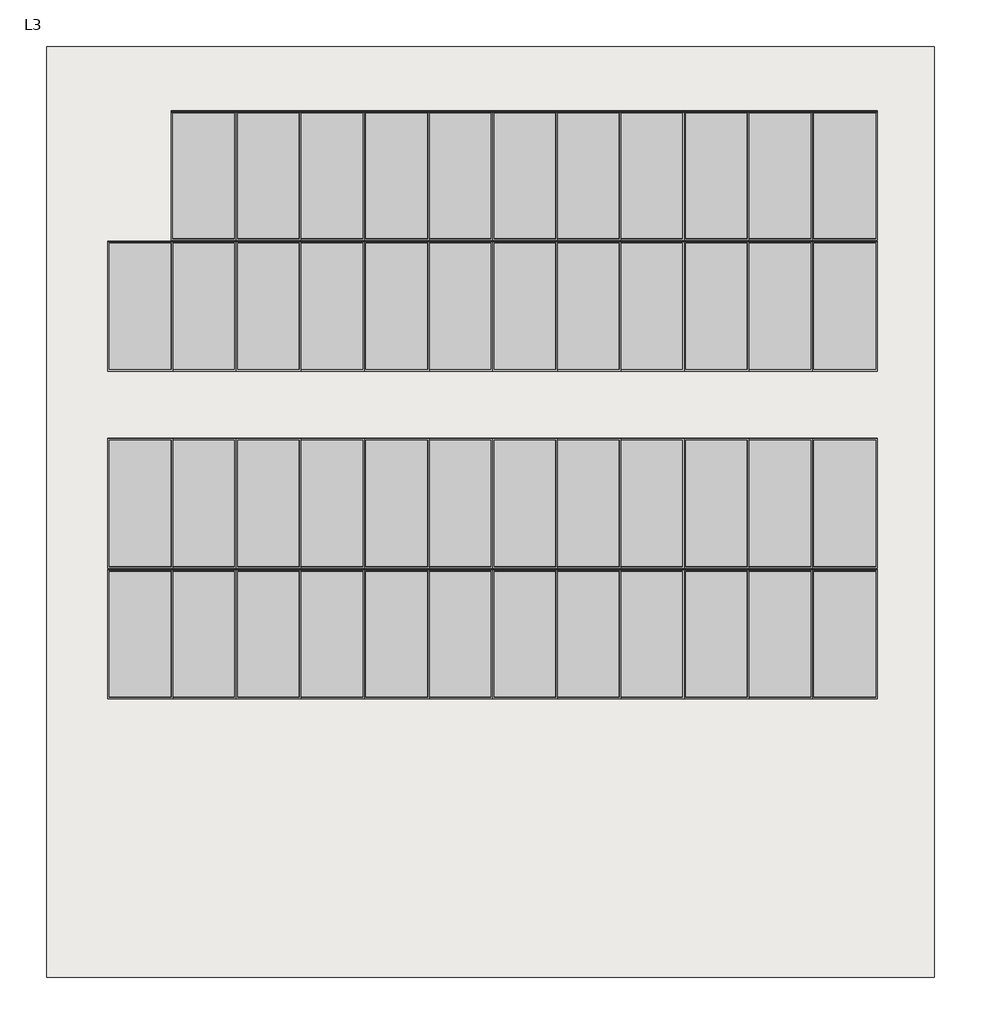
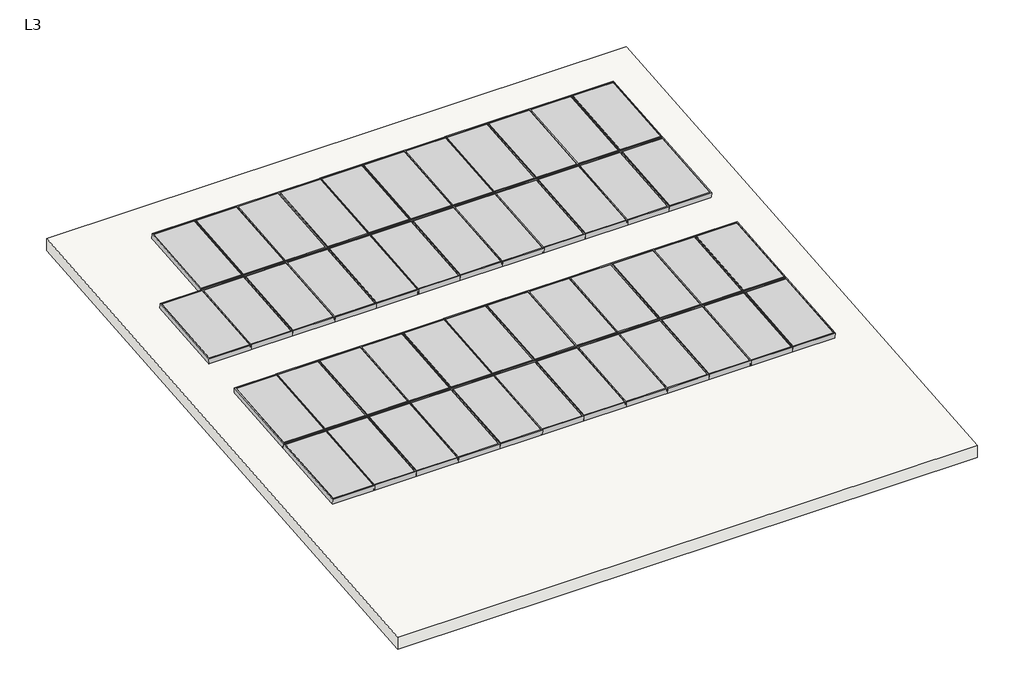
# One storey: 47 proxies, 1 roof.
"""IFC4 building model written with IfcOpenShell, lengths in millimetres."""

import ifcopenshell
import ifcopenshell.guid

model = None  # the IFC model being written
_history = None  # IfcOwnerHistory: only IFC2X3 demands one
_inside = {}  # id of a spatial element -> (the spatial element, [elements in it])
_under = {}  # id of a project, library or spatial element -> (it, [spatial elements below it])
_declared = {}  # id of a project -> (the project, [libraries it declares])
_typed = {}  # id of a type object -> (the type object, [elements of that type])
_made_of = {}  # id of a material, layer set ... -> (it, [elements and type objects made of it])


def new_model(schema):
    """Start an empty IFC model of exactly this schema.

    Asked for "IFC4X3", IfcOpenShell would pick the latest addendum, in which some entities
    have other attributes; the version numbers below select the first issue.
    IFC2X3 requires an IfcOwnerHistory on every rooted entity: one is made here for all.
    """
    global model, _history
    if schema == "IFC4X3":
        model = ifcopenshell.file(schema_version=(4, 3, 0, 0))
    else:
        model = ifcopenshell.file(schema=schema)
    _inside.clear()
    _under.clear()
    _declared.clear()
    _typed.clear()
    _made_of.clear()
    _history = None
    if model.schema == "IFC2X3":
        org = make("IfcOrganization", Name="unknown")
        user = make(
            "IfcPersonAndOrganization",
            ThePerson=make("IfcPerson", FamilyName="unknown"),
            TheOrganization=org,
        )
        app = make(
            "IfcApplication",
            ApplicationDeveloper=org,
            Version="unknown",
            ApplicationFullName="unknown",
            ApplicationIdentifier="unknown",
        )
        _history = make(
            "IfcOwnerHistory",
            OwningUser=user,
            OwningApplication=app,
            ChangeAction="ADDED",
            CreationDate=0,
        )
    return model


def make(cls, **values):
    """One entity of the class cls with the attributes given. An attribute that is None is left unset."""
    return model.create_entity(
        cls, **{name: value for name, value in values.items() if value is not None}
    )


def rooted(cls, **values):
    """An entity with a GlobalId (a new one), such as an element, a storey or a relation."""
    return make(cls, GlobalId=ifcopenshell.guid.new(), OwnerHistory=_history, **values)


def si_unit(unit_type, name, prefix=None):
    """IfcSIUnit, for example si_unit("LENGTHUNIT", "METRE", prefix="MILLI")."""
    return make("IfcSIUnit", UnitType=unit_type, Prefix=prefix, Name=name)


def assignment(units):
    """IfcUnitAssignment: the units of a project."""
    return None if units is None else make("IfcUnitAssignment", Units=units)


def point(xyz):
    """IfcCartesianPoint."""
    return None if xyz is None else make("IfcCartesianPoint", Coordinates=xyz)


def direction(xyz):
    """IfcDirection."""
    return None if xyz is None else make("IfcDirection", DirectionRatios=xyz)


def frame(location, z_axis=None, x_axis=None):
    """IfcAxis2Placement3D, a coordinate frame: its origin and axes. An axis left out is left unset."""
    return make(
        "IfcAxis2Placement3D",
        Location=point(location),
        Axis=direction(z_axis),
        RefDirection=direction(x_axis),
    )


def origin():
    """The frame at (0, 0, 0) with its axes left unset."""
    return frame((0.0, 0.0, 0.0))


def origin_with_axes():
    """The frame at (0, 0, 0) with the z axis (0, 0, 1) and the x axis (1, 0, 0) written out."""
    return frame((0.0, 0.0, 0.0), z_axis=(0.0, 0.0, 1.0), x_axis=(1.0, 0.0, 0.0))


def place(relative_to, where):
    """IfcLocalPlacement: puts the frame where relative to a parent placement (None: the world)."""
    return make(
        "IfcLocalPlacement", PlacementRelTo=relative_to, RelativePlacement=where
    )


def context(
    kind, dimensions, precision=None, world=None, true_north=None, identifier=None
):
    """IfcGeometricRepresentationContext, for example the 3D "Model" context."""
    return make(
        "IfcGeometricRepresentationContext",
        ContextIdentifier=identifier,
        ContextType=kind,
        CoordinateSpaceDimension=dimensions,
        Precision=precision,
        WorldCoordinateSystem=world,
        TrueNorth=true_north,
    )


def project(units=None, contexts=None):
    """IfcProject with its units and contexts."""
    return rooted(
        "IfcProject",
        Name="project",
        RepresentationContexts=contexts,
        UnitsInContext=assignment(units),
    )


def spatial(cls, under=None, at=None, **own):
    """A site, building, storey or space (cls), placed at a placement, below another one or the project."""
    s = rooted(cls, ObjectPlacement=at, **own)
    if under is not None:
        _under.setdefault(under.id(), (under, []))[1].append(s)
    return s


def polyline(points):
    """IfcPolyline through the points."""
    return make("IfcPolyline", Points=[point(p) for p in points])


def outline(outer, holes=None, kind="AREA"):
    """IfcArbitraryClosedProfileDef: a profile drawn as a closed curve; with holes, ...WithVoids."""
    if holes is None:
        return make("IfcArbitraryClosedProfileDef", ProfileType=kind, OuterCurve=outer)
    return make(
        "IfcArbitraryProfileDefWithVoids",
        ProfileType=kind,
        OuterCurve=outer,
        InnerCurves=holes,
    )


def extrude(swept, where, along, depth):
    """IfcExtrudedAreaSolid: the profile swept, set in the frame where, extruded along a direction by depth."""
    return make(
        "IfcExtrudedAreaSolid",
        SweptArea=swept,
        Position=where,
        ExtrudedDirection=direction(along),
        Depth=depth,
    )


def shape(context_of_items, identifier, shape_type, items):
    """IfcShapeRepresentation: the items that make up one representation, for example the "Body"."""
    return make(
        "IfcShapeRepresentation",
        ContextOfItems=context_of_items,
        RepresentationIdentifier=identifier,
        RepresentationType=shape_type,
        Items=items,
    )


def source(mapping_origin, context_of_items, identifier, shape_type, items):
    """IfcRepresentationMap: a shape defined once, which mapped items show again and again."""
    return make(
        "IfcRepresentationMap",
        MappingOrigin=mapping_origin,
        MappedRepresentation=shape(context_of_items, identifier, shape_type, items),
    )


def transform(
    local_origin,
    x_axis=None,
    y_axis=None,
    z_axis=None,
    scale=None,
    scale2=None,
    scale3=None,
    uniform=True,
):
    """IfcCartesianTransformationOperator3D, or its non-uniform kind. x_axis, y_axis, z_axis: its Axis1, 2, 3."""
    if uniform:
        return make(
            "IfcCartesianTransformationOperator3D",
            Axis1=direction(x_axis),
            Axis2=direction(y_axis),
            LocalOrigin=point(local_origin),
            Scale=scale,
            Axis3=direction(z_axis),
        )
    return make(
        "IfcCartesianTransformationOperator3DnonUniform",
        Axis1=direction(x_axis),
        Axis2=direction(y_axis),
        LocalOrigin=point(local_origin),
        Scale=scale,
        Axis3=direction(z_axis),
        Scale2=scale2,
        Scale3=scale3,
    )


def mapped(mapping_source, mapping_target):
    """IfcMappedItem: shows the shape of a source again, moved by a transform."""
    return make(
        "IfcMappedItem", MappingSource=mapping_source, MappingTarget=mapping_target
    )


def made_of(thing, what):
    """Note that an element or type object is made of a material, layer set ...; save() writes the relation."""
    if what is not None:
        _made_of.setdefault(what.id(), (what, []))[1].append(thing)
    return thing


def element(
    cls,
    number,
    at=None,
    inside=None,
    cuts=None,
    type_object=None,
    material=None,
    context=None,
    identifier="Body",
    shape_type=None,
    held_by="IfcProductDefinitionShape",
    body=None,
    shapes=None,
    **own,
):
    """One element of the class cls, such as IfcWall. Its Tag is "e" and its number.

    at: its placement. inside: the storey or other place that contains it. cuts: it is an
    opening in that element (IfcRelVoidsElement). A single representation is given by context,
    identifier, shape_type and body (its items); several are given by shapes. held_by: the class
    of the entity that holds the representations. save() writes the other relations.
    """
    e = rooted(cls, Tag="e%d" % number, ObjectPlacement=at, **own)
    if body is not None:
        shapes = [shape(context, identifier, shape_type, body)]
    if shapes is not None:
        e.Representation = make(held_by, Representations=shapes)
    if inside is not None:
        _inside.setdefault(inside.id(), (inside, []))[1].append(e)
    if cuts is not None:
        rooted(
            "IfcRelVoidsElement", RelatingBuildingElement=cuts, RelatedOpeningElement=e
        )
    if type_object is not None:
        _typed.setdefault(type_object.id(), (type_object, []))[1].append(e)
    return made_of(e, material)


def aggregate(whole, parts):
    """IfcRelAggregates: a whole, such as a stair, and the parts it consists of."""
    return rooted("IfcRelAggregates", RelatingObject=whole, RelatedObjects=parts)


def save(model, path):
    """Write the relations noted so far, then the file.

    IfcRelAggregates (storeys below a building ...), IfcRelContainedInSpatialStructure (elements
    in a storey), IfcRelDefinesByType, IfcRelAssociatesMaterial and IfcRelDeclares: one each for
    every whole, place, type object, material and project.
    """
    for whole, parts in _under.values():
        aggregate(whole, parts)
    for where, things in _inside.values():
        rooted(
            "IfcRelContainedInSpatialStructure",
            RelatedElements=things,
            RelatingStructure=where,
        )
    for kind, things in _typed.values():
        rooted("IfcRelDefinesByType", RelatedObjects=things, RelatingType=kind)
    for what, things in _made_of.values():
        rooted("IfcRelAssociatesMaterial", RelatedObjects=things, RelatingMaterial=what)
    for by, libraries in _declared.values():
        rooted("IfcRelDeclares", RelatingContext=by, RelatedDefinitions=libraries)
    model.write(path)


def m_solar_panel_750_x_1500mm_21fb4d5c(model_context):
    return source(origin(), model_context, "Body", "SweptSolid", [
        extrude(outline(polyline([(32.32, 1500.0), (782.32, 1500.0), (782.32, 0.0), (32.32, 0.0), (32.32, 1500.0)]), holes=[polyline([(763.27, 1480.95), (51.37, 1480.95), (51.37, 19.05), (763.27, 19.05), (763.27, 1480.95)])]), origin_with_axes(), (0.0, 0.0, 1.0), 100.0),
        extrude(outline(polyline([(763.27, 1480.95), (763.27, 19.05), (51.37, 19.05), (51.37, 1480.95), (763.27, 1480.95)])), origin_with_axes(), (0.0, 0.0, 1.0), 93.65),
    ])


model = new_model("IFC4")

# Units and contexts
model_context = context("Model", 3, world=origin())
ifc_project = project(units=[si_unit("LENGTHUNIT", "METRE", prefix="MILLI")], contexts=[model_context])

# Site, building, storey
site = spatial("IfcSite", under=ifc_project)
building = spatial("IfcBuilding", under=site)
storey = spatial("IfcBuildingStorey", under=building, Name="L3", Elevation=6000.0)

# Proxies
placement = place(None, origin())
m_solar_panel_750_x_1500mm_shape = m_solar_panel_750_x_1500mm_21fb4d5c(model_context)
element("IfcBuildingElementProxy", 1, Name="M_Solar Panel : 750 x 1500mm", ObjectType="M_Solar Panel : 750 x 1500mm", at=placement, inside=storey, context=model_context, shape_type="MappedRepresentation", body=[
    mapped(m_solar_panel_750_x_1500mm_shape, transform((-3719.703333, 2644.8337429, 6971.2483311), x_axis=(1.0, 0.0, 0.0), y_axis=(0.0, 0.9961946980917455, 0.08715574274765815), z_axis=(0.0, -0.08715574274765815, 0.9961946980917455))),
])
element("IfcBuildingElementProxy", 2, Name="M_Solar Panel : 750 x 1500mm", ObjectType="M_Solar Panel : 750 x 1500mm", at=placement, inside=storey, context=model_context, shape_type="MappedRepresentation", body=[
    mapped(m_solar_panel_750_x_1500mm_shape, transform((-2969.703333, 2644.8337429, 6971.2483311), x_axis=(1.0, 0.0, 0.0), y_axis=(0.0, 0.9961946980917455, 0.08715574274765815), z_axis=(0.0, -0.08715574274765815, 0.9961946980917455))),
])
element("IfcBuildingElementProxy", 3, Name="M_Solar Panel : 750 x 1500mm", ObjectType="M_Solar Panel : 750 x 1500mm", at=placement, inside=storey, context=model_context, shape_type="MappedRepresentation", body=[
    mapped(m_solar_panel_750_x_1500mm_shape, transform((-2238.753333, 2644.8337429, 6971.2483311), x_axis=(1.0, 0.0, 0.0), y_axis=(0.0, 0.9961946980917455, 0.08715574274765815), z_axis=(0.0, -0.08715574274765815, 0.9961946980917455))),
])
element("IfcBuildingElementProxy", 4, Name="M_Solar Panel : 750 x 1500mm", ObjectType="M_Solar Panel : 750 x 1500mm", at=placement, inside=storey, context=model_context, shape_type="MappedRepresentation", body=[
    mapped(m_solar_panel_750_x_1500mm_shape, transform((-1488.753333, 2644.8337429, 6971.2483311), x_axis=(1.0, 0.0, 0.0), y_axis=(0.0, 0.9961946980917455, 0.08715574274765815), z_axis=(0.0, -0.08715574274765815, 0.9961946980917455))),
])
element("IfcBuildingElementProxy", 5, Name="M_Solar Panel : 750 x 1500mm", ObjectType="M_Solar Panel : 750 x 1500mm", at=placement, inside=storey, context=model_context, shape_type="MappedRepresentation", body=[
    mapped(m_solar_panel_750_x_1500mm_shape, transform((-757.803333, 2644.8337429, 6971.2483311), x_axis=(1.0, 0.0, 0.0), y_axis=(0.0, 0.9961946980917455, 0.08715574274765815), z_axis=(0.0, -0.08715574274765815, 0.9961946980917455))),
])
element("IfcBuildingElementProxy", 6, Name="M_Solar Panel : 750 x 1500mm", ObjectType="M_Solar Panel : 750 x 1500mm", at=placement, inside=storey, context=model_context, shape_type="MappedRepresentation", body=[
    mapped(m_solar_panel_750_x_1500mm_shape, transform((-7.803333, 2644.8337429, 6971.2483311), x_axis=(1.0, 0.0, 0.0), y_axis=(0.0, 0.9961946980917455, 0.08715574274765815), z_axis=(0.0, -0.08715574274765815, 0.9961946980917455))),
])
element("IfcBuildingElementProxy", 7, Name="M_Solar Panel : 750 x 1500mm", ObjectType="M_Solar Panel : 750 x 1500mm", at=placement, inside=storey, context=model_context, shape_type="MappedRepresentation", body=[
    mapped(m_solar_panel_750_x_1500mm_shape, transform((723.146667, 2644.8337429, 6971.2483311), x_axis=(1.0, 0.0, 0.0), y_axis=(0.0, 0.9961946980917455, 0.08715574274765815), z_axis=(0.0, -0.08715574274765815, 0.9961946980917455))),
])
element("IfcBuildingElementProxy", 8, Name="M_Solar Panel : 750 x 1500mm", ObjectType="M_Solar Panel : 750 x 1500mm", at=placement, inside=storey, context=model_context, shape_type="MappedRepresentation", body=[
    mapped(m_solar_panel_750_x_1500mm_shape, transform((1454.096667, 2644.8337429, 6971.2483311), x_axis=(1.0, 0.0, 0.0), y_axis=(0.0, 0.9961946980917455, 0.08715574274765815), z_axis=(0.0, -0.08715574274765815, 0.9961946980917455))),
])
element("IfcBuildingElementProxy", 9, Name="M_Solar Panel : 750 x 1500mm", ObjectType="M_Solar Panel : 750 x 1500mm", at=placement, inside=storey, context=model_context, shape_type="MappedRepresentation", body=[
    mapped(m_solar_panel_750_x_1500mm_shape, transform((2204.096667, 2644.8337429, 6971.2483311), x_axis=(1.0, 0.0, 0.0), y_axis=(0.0, 0.9961946980917455, 0.08715574274765815), z_axis=(0.0, -0.08715574274765815, 0.9961946980917455))),
])
element("IfcBuildingElementProxy", 10, Name="M_Solar Panel : 750 x 1500mm", ObjectType="M_Solar Panel : 750 x 1500mm", at=placement, inside=storey, context=model_context, shape_type="MappedRepresentation", body=[
    mapped(m_solar_panel_750_x_1500mm_shape, transform((2935.046667, 2644.8337429, 6971.2483311), x_axis=(1.0, 0.0, 0.0), y_axis=(0.0, 0.9961946980917455, 0.08715574274765815), z_axis=(0.0, -0.08715574274765815, 0.9961946980917455))),
])
element("IfcBuildingElementProxy", 11, Name="M_Solar Panel : 750 x 1500mm", ObjectType="M_Solar Panel : 750 x 1500mm", at=placement, inside=storey, context=model_context, shape_type="MappedRepresentation", body=[
    mapped(m_solar_panel_750_x_1500mm_shape, transform((3685.046667, 2644.8337429, 6971.2483311), x_axis=(1.0, 0.0, 0.0), y_axis=(0.0, 0.9961946980917455, 0.08715574274765815), z_axis=(0.0, -0.08715574274765815, 0.9961946980917455))),
])
element("IfcBuildingElementProxy", 12, Name="M_Solar Panel : 750 x 1500mm", ObjectType="M_Solar Panel : 750 x 1500mm", at=placement, inside=storey, context=model_context, shape_type="MappedRepresentation", body=[
    mapped(m_solar_panel_750_x_1500mm_shape, transform((-4450.653333, 1135.5987753, 6839.2073808), x_axis=(1.0, 0.0, 0.0), y_axis=(0.0, 0.9961946980917455, 0.08715574274765815), z_axis=(0.0, -0.08715574274765815, 0.9961946980917455))),
])
element("IfcBuildingElementProxy", 13, Name="M_Solar Panel : 750 x 1500mm", ObjectType="M_Solar Panel : 750 x 1500mm", at=placement, inside=storey, context=model_context, shape_type="MappedRepresentation", body=[
    mapped(m_solar_panel_750_x_1500mm_shape, transform((-3719.703333, 1135.5987753, 6839.2073808), x_axis=(1.0, 0.0, 0.0), y_axis=(0.0, 0.9961946980917455, 0.08715574274765815), z_axis=(0.0, -0.08715574274765815, 0.9961946980917455))),
])
element("IfcBuildingElementProxy", 14, Name="M_Solar Panel : 750 x 1500mm", ObjectType="M_Solar Panel : 750 x 1500mm", at=placement, inside=storey, context=model_context, shape_type="MappedRepresentation", body=[
    mapped(m_solar_panel_750_x_1500mm_shape, transform((-2969.703333, 1135.5987753, 6839.2073808), x_axis=(1.0, 0.0, 0.0), y_axis=(0.0, 0.9961946980917455, 0.08715574274765815), z_axis=(0.0, -0.08715574274765815, 0.9961946980917455))),
])
element("IfcBuildingElementProxy", 15, Name="M_Solar Panel : 750 x 1500mm", ObjectType="M_Solar Panel : 750 x 1500mm", at=placement, inside=storey, context=model_context, shape_type="MappedRepresentation", body=[
    mapped(m_solar_panel_750_x_1500mm_shape, transform((-2238.753333, 1135.5987753, 6839.2073808), x_axis=(1.0, 0.0, 0.0), y_axis=(0.0, 0.9961946980917455, 0.08715574274765815), z_axis=(0.0, -0.08715574274765815, 0.9961946980917455))),
])
element("IfcBuildingElementProxy", 16, Name="M_Solar Panel : 750 x 1500mm", ObjectType="M_Solar Panel : 750 x 1500mm", at=placement, inside=storey, context=model_context, shape_type="MappedRepresentation", body=[
    mapped(m_solar_panel_750_x_1500mm_shape, transform((-1488.753333, 1135.5987753, 6839.2073808), x_axis=(1.0, 0.0, 0.0), y_axis=(0.0, 0.9961946980917455, 0.08715574274765815), z_axis=(0.0, -0.08715574274765815, 0.9961946980917455))),
])
element("IfcBuildingElementProxy", 17, Name="M_Solar Panel : 750 x 1500mm", ObjectType="M_Solar Panel : 750 x 1500mm", at=placement, inside=storey, context=model_context, shape_type="MappedRepresentation", body=[
    mapped(m_solar_panel_750_x_1500mm_shape, transform((-757.803333, 1135.5987753, 6839.2073808), x_axis=(1.0, 0.0, 0.0), y_axis=(0.0, 0.9961946980917455, 0.08715574274765815), z_axis=(0.0, -0.08715574274765815, 0.9961946980917455))),
])
element("IfcBuildingElementProxy", 18, Name="M_Solar Panel : 750 x 1500mm", ObjectType="M_Solar Panel : 750 x 1500mm", at=placement, inside=storey, context=model_context, shape_type="MappedRepresentation", body=[
    mapped(m_solar_panel_750_x_1500mm_shape, transform((-7.803333, 1135.5987753, 6839.2073808), x_axis=(1.0, 0.0, 0.0), y_axis=(0.0, 0.9961946980917455, 0.08715574274765815), z_axis=(0.0, -0.08715574274765815, 0.9961946980917455))),
])
element("IfcBuildingElementProxy", 19, Name="M_Solar Panel : 750 x 1500mm", ObjectType="M_Solar Panel : 750 x 1500mm", at=placement, inside=storey, context=model_context, shape_type="MappedRepresentation", body=[
    mapped(m_solar_panel_750_x_1500mm_shape, transform((723.146667, 1135.5987753, 6839.2073808), x_axis=(1.0, 0.0, 0.0), y_axis=(0.0, 0.9961946980917455, 0.08715574274765815), z_axis=(0.0, -0.08715574274765815, 0.9961946980917455))),
])
element("IfcBuildingElementProxy", 20, Name="M_Solar Panel : 750 x 1500mm", ObjectType="M_Solar Panel : 750 x 1500mm", at=placement, inside=storey, context=model_context, shape_type="MappedRepresentation", body=[
    mapped(m_solar_panel_750_x_1500mm_shape, transform((1454.096667, 1135.5987753, 6839.2073808), x_axis=(1.0, 0.0, 0.0), y_axis=(0.0, 0.9961946980917455, 0.08715574274765815), z_axis=(0.0, -0.08715574274765815, 0.9961946980917455))),
])
element("IfcBuildingElementProxy", 21, Name="M_Solar Panel : 750 x 1500mm", ObjectType="M_Solar Panel : 750 x 1500mm", at=placement, inside=storey, context=model_context, shape_type="MappedRepresentation", body=[
    mapped(m_solar_panel_750_x_1500mm_shape, transform((2204.096667, 1135.5987753, 6839.2073808), x_axis=(1.0, 0.0, 0.0), y_axis=(0.0, 0.9961946980917455, 0.08715574274765815), z_axis=(0.0, -0.08715574274765815, 0.9961946980917455))),
])
element("IfcBuildingElementProxy", 22, Name="M_Solar Panel : 750 x 1500mm", ObjectType="M_Solar Panel : 750 x 1500mm", at=placement, inside=storey, context=model_context, shape_type="MappedRepresentation", body=[
    mapped(m_solar_panel_750_x_1500mm_shape, transform((2935.046667, 1135.5987753, 6839.2073808), x_axis=(1.0, 0.0, 0.0), y_axis=(0.0, 0.9961946980917455, 0.08715574274765815), z_axis=(0.0, -0.08715574274765815, 0.9961946980917455))),
])
element("IfcBuildingElementProxy", 23, Name="M_Solar Panel : 750 x 1500mm", ObjectType="M_Solar Panel : 750 x 1500mm", at=placement, inside=storey, context=model_context, shape_type="MappedRepresentation", body=[
    mapped(m_solar_panel_750_x_1500mm_shape, transform((3685.046667, 1135.5987753, 6839.2073808), x_axis=(1.0, 0.0, 0.0), y_axis=(0.0, 0.9961946980917455, 0.08715574274765815), z_axis=(0.0, -0.08715574274765815, 0.9961946980917455))),
])
element("IfcBuildingElementProxy", 24, Name="M_Solar Panel : 750 x 1500mm", ObjectType="M_Solar Panel : 750 x 1500mm", at=placement, inside=storey, context=model_context, shape_type="MappedRepresentation", body=[
    mapped(m_solar_panel_750_x_1500mm_shape, transform((-4450.653333, -1140.7061098, 6640.0565086), x_axis=(1.0, 0.0, 0.0), y_axis=(0.0, 0.9961946980917455, 0.08715574274765815), z_axis=(0.0, -0.08715574274765815, 0.9961946980917455))),
])
element("IfcBuildingElementProxy", 25, Name="M_Solar Panel : 750 x 1500mm", ObjectType="M_Solar Panel : 750 x 1500mm", at=placement, inside=storey, context=model_context, shape_type="MappedRepresentation", body=[
    mapped(m_solar_panel_750_x_1500mm_shape, transform((-3719.703333, -1140.7061098, 6640.0565086), x_axis=(1.0, 0.0, 0.0), y_axis=(0.0, 0.9961946980917455, 0.08715574274765815), z_axis=(0.0, -0.08715574274765815, 0.9961946980917455))),
])
element("IfcBuildingElementProxy", 26, Name="M_Solar Panel : 750 x 1500mm", ObjectType="M_Solar Panel : 750 x 1500mm", at=placement, inside=storey, context=model_context, shape_type="MappedRepresentation", body=[
    mapped(m_solar_panel_750_x_1500mm_shape, transform((-2969.703333, -1140.7061098, 6640.0565086), x_axis=(1.0, 0.0, 0.0), y_axis=(0.0, 0.9961946980917455, 0.08715574274765815), z_axis=(0.0, -0.08715574274765815, 0.9961946980917455))),
])
element("IfcBuildingElementProxy", 27, Name="M_Solar Panel : 750 x 1500mm", ObjectType="M_Solar Panel : 750 x 1500mm", at=placement, inside=storey, context=model_context, shape_type="MappedRepresentation", body=[
    mapped(m_solar_panel_750_x_1500mm_shape, transform((-2238.753333, -1140.7061098, 6640.0565086), x_axis=(1.0, 0.0, 0.0), y_axis=(0.0, 0.9961946980917455, 0.08715574274765815), z_axis=(0.0, -0.08715574274765815, 0.9961946980917455))),
])
element("IfcBuildingElementProxy", 28, Name="M_Solar Panel : 750 x 1500mm", ObjectType="M_Solar Panel : 750 x 1500mm", at=placement, inside=storey, context=model_context, shape_type="MappedRepresentation", body=[
    mapped(m_solar_panel_750_x_1500mm_shape, transform((-1488.753333, -1140.7061098, 6640.0565086), x_axis=(1.0, 0.0, 0.0), y_axis=(0.0, 0.9961946980917455, 0.08715574274765815), z_axis=(0.0, -0.08715574274765815, 0.9961946980917455))),
])
element("IfcBuildingElementProxy", 29, Name="M_Solar Panel : 750 x 1500mm", ObjectType="M_Solar Panel : 750 x 1500mm", at=placement, inside=storey, context=model_context, shape_type="MappedRepresentation", body=[
    mapped(m_solar_panel_750_x_1500mm_shape, transform((-757.803333, -1140.7061098, 6640.0565086), x_axis=(1.0, 0.0, 0.0), y_axis=(0.0, 0.9961946980917455, 0.08715574274765815), z_axis=(0.0, -0.08715574274765815, 0.9961946980917455))),
])
element("IfcBuildingElementProxy", 30, Name="M_Solar Panel : 750 x 1500mm", ObjectType="M_Solar Panel : 750 x 1500mm", at=placement, inside=storey, context=model_context, shape_type="MappedRepresentation", body=[
    mapped(m_solar_panel_750_x_1500mm_shape, transform((-7.803333, -1140.7061098, 6640.0565086), x_axis=(1.0, 0.0, 0.0), y_axis=(0.0, 0.9961946980917455, 0.08715574274765815), z_axis=(0.0, -0.08715574274765815, 0.9961946980917455))),
])
element("IfcBuildingElementProxy", 31, Name="M_Solar Panel : 750 x 1500mm", ObjectType="M_Solar Panel : 750 x 1500mm", at=placement, inside=storey, context=model_context, shape_type="MappedRepresentation", body=[
    mapped(m_solar_panel_750_x_1500mm_shape, transform((723.146667, -1140.7061098, 6640.0565086), x_axis=(1.0, 0.0, 0.0), y_axis=(0.0, 0.9961946980917455, 0.08715574274765815), z_axis=(0.0, -0.08715574274765815, 0.9961946980917455))),
])
element("IfcBuildingElementProxy", 32, Name="M_Solar Panel : 750 x 1500mm", ObjectType="M_Solar Panel : 750 x 1500mm", at=placement, inside=storey, context=model_context, shape_type="MappedRepresentation", body=[
    mapped(m_solar_panel_750_x_1500mm_shape, transform((1454.096667, -1140.7061098, 6640.0565086), x_axis=(1.0, 0.0, 0.0), y_axis=(0.0, 0.9961946980917455, 0.08715574274765815), z_axis=(0.0, -0.08715574274765815, 0.9961946980917455))),
])
element("IfcBuildingElementProxy", 33, Name="M_Solar Panel : 750 x 1500mm", ObjectType="M_Solar Panel : 750 x 1500mm", at=placement, inside=storey, context=model_context, shape_type="MappedRepresentation", body=[
    mapped(m_solar_panel_750_x_1500mm_shape, transform((2204.096667, -1140.7061098, 6640.0565086), x_axis=(1.0, 0.0, 0.0), y_axis=(0.0, 0.9961946980917455, 0.08715574274765815), z_axis=(0.0, -0.08715574274765815, 0.9961946980917455))),
])
element("IfcBuildingElementProxy", 34, Name="M_Solar Panel : 750 x 1500mm", ObjectType="M_Solar Panel : 750 x 1500mm", at=placement, inside=storey, context=model_context, shape_type="MappedRepresentation", body=[
    mapped(m_solar_panel_750_x_1500mm_shape, transform((2935.046667, -1140.7061098, 6640.0565086), x_axis=(1.0, 0.0, 0.0), y_axis=(0.0, 0.9961946980917455, 0.08715574274765815), z_axis=(0.0, -0.08715574274765815, 0.9961946980917455))),
])
element("IfcBuildingElementProxy", 35, Name="M_Solar Panel : 750 x 1500mm", ObjectType="M_Solar Panel : 750 x 1500mm", at=placement, inside=storey, context=model_context, shape_type="MappedRepresentation", body=[
    mapped(m_solar_panel_750_x_1500mm_shape, transform((3685.046667, -1140.7061098, 6640.0565086), x_axis=(1.0, 0.0, 0.0), y_axis=(0.0, 0.9961946980917455, 0.08715574274765815), z_axis=(0.0, -0.08715574274765815, 0.9961946980917455))),
])
element("IfcBuildingElementProxy", 36, Name="M_Solar Panel : 750 x 1500mm", ObjectType="M_Solar Panel : 750 x 1500mm", at=placement, inside=storey, context=model_context, shape_type="MappedRepresentation", body=[
    mapped(m_solar_panel_750_x_1500mm_shape, transform((-4450.653333, -2649.9410774, 6508.0155584), x_axis=(1.0, 0.0, 0.0), y_axis=(0.0, 0.9961946980917455, 0.08715574274765815), z_axis=(0.0, -0.08715574274765815, 0.9961946980917455))),
])
element("IfcBuildingElementProxy", 37, Name="M_Solar Panel : 750 x 1500mm", ObjectType="M_Solar Panel : 750 x 1500mm", at=placement, inside=storey, context=model_context, shape_type="MappedRepresentation", body=[
    mapped(m_solar_panel_750_x_1500mm_shape, transform((-3719.703333, -2649.9410774, 6508.0155584), x_axis=(1.0, 0.0, 0.0), y_axis=(0.0, 0.9961946980917455, 0.08715574274765815), z_axis=(0.0, -0.08715574274765815, 0.9961946980917455))),
])
element("IfcBuildingElementProxy", 38, Name="M_Solar Panel : 750 x 1500mm", ObjectType="M_Solar Panel : 750 x 1500mm", at=placement, inside=storey, context=model_context, shape_type="MappedRepresentation", body=[
    mapped(m_solar_panel_750_x_1500mm_shape, transform((-2969.703333, -2649.9410774, 6508.0155584), x_axis=(1.0, 0.0, 0.0), y_axis=(0.0, 0.9961946980917455, 0.08715574274765815), z_axis=(0.0, -0.08715574274765815, 0.9961946980917455))),
])
element("IfcBuildingElementProxy", 39, Name="M_Solar Panel : 750 x 1500mm", ObjectType="M_Solar Panel : 750 x 1500mm", at=placement, inside=storey, context=model_context, shape_type="MappedRepresentation", body=[
    mapped(m_solar_panel_750_x_1500mm_shape, transform((-2238.753333, -2649.9410774, 6508.0155584), x_axis=(1.0, 0.0, 0.0), y_axis=(0.0, 0.9961946980917455, 0.08715574274765815), z_axis=(0.0, -0.08715574274765815, 0.9961946980917455))),
])
element("IfcBuildingElementProxy", 40, Name="M_Solar Panel : 750 x 1500mm", ObjectType="M_Solar Panel : 750 x 1500mm", at=placement, inside=storey, context=model_context, shape_type="MappedRepresentation", body=[
    mapped(m_solar_panel_750_x_1500mm_shape, transform((-1488.753333, -2649.9410774, 6508.0155584), x_axis=(1.0, 0.0, 0.0), y_axis=(0.0, 0.9961946980917455, 0.08715574274765815), z_axis=(0.0, -0.08715574274765815, 0.9961946980917455))),
])
element("IfcBuildingElementProxy", 41, Name="M_Solar Panel : 750 x 1500mm", ObjectType="M_Solar Panel : 750 x 1500mm", at=placement, inside=storey, context=model_context, shape_type="MappedRepresentation", body=[
    mapped(m_solar_panel_750_x_1500mm_shape, transform((-757.803333, -2649.9410774, 6508.0155584), x_axis=(1.0, 0.0, 0.0), y_axis=(0.0, 0.9961946980917455, 0.08715574274765815), z_axis=(0.0, -0.08715574274765815, 0.9961946980917455))),
])
element("IfcBuildingElementProxy", 42, Name="M_Solar Panel : 750 x 1500mm", ObjectType="M_Solar Panel : 750 x 1500mm", at=placement, inside=storey, context=model_context, shape_type="MappedRepresentation", body=[
    mapped(m_solar_panel_750_x_1500mm_shape, transform((-7.803333, -2649.9410774, 6508.0155584), x_axis=(1.0, 0.0, 0.0), y_axis=(0.0, 0.9961946980917455, 0.08715574274765815), z_axis=(0.0, -0.08715574274765815, 0.9961946980917455))),
])
element("IfcBuildingElementProxy", 43, Name="M_Solar Panel : 750 x 1500mm", ObjectType="M_Solar Panel : 750 x 1500mm", at=placement, inside=storey, context=model_context, shape_type="MappedRepresentation", body=[
    mapped(m_solar_panel_750_x_1500mm_shape, transform((723.146667, -2649.9410774, 6508.0155584), x_axis=(1.0, 0.0, 0.0), y_axis=(0.0, 0.9961946980917455, 0.08715574274765815), z_axis=(0.0, -0.08715574274765815, 0.9961946980917455))),
])
element("IfcBuildingElementProxy", 44, Name="M_Solar Panel : 750 x 1500mm", ObjectType="M_Solar Panel : 750 x 1500mm", at=placement, inside=storey, context=model_context, shape_type="MappedRepresentation", body=[
    mapped(m_solar_panel_750_x_1500mm_shape, transform((1454.096667, -2649.9410774, 6508.0155584), x_axis=(1.0, 0.0, 0.0), y_axis=(0.0, 0.9961946980917455, 0.08715574274765815), z_axis=(0.0, -0.08715574274765815, 0.9961946980917455))),
])
element("IfcBuildingElementProxy", 45, Name="M_Solar Panel : 750 x 1500mm", ObjectType="M_Solar Panel : 750 x 1500mm", at=placement, inside=storey, context=model_context, shape_type="MappedRepresentation", body=[
    mapped(m_solar_panel_750_x_1500mm_shape, transform((2204.096667, -2649.9410774, 6508.0155584), x_axis=(1.0, 0.0, 0.0), y_axis=(0.0, 0.9961946980917455, 0.08715574274765815), z_axis=(0.0, -0.08715574274765815, 0.9961946980917455))),
])
element("IfcBuildingElementProxy", 46, Name="M_Solar Panel : 750 x 1500mm", ObjectType="M_Solar Panel : 750 x 1500mm", at=placement, inside=storey, context=model_context, shape_type="MappedRepresentation", body=[
    mapped(m_solar_panel_750_x_1500mm_shape, transform((2935.046667, -2649.9410774, 6508.0155584), x_axis=(1.0, 0.0, 0.0), y_axis=(0.0, 0.9961946980917455, 0.08715574274765815), z_axis=(0.0, -0.08715574274765815, 0.9961946980917455))),
])
element("IfcBuildingElementProxy", 47, Name="M_Solar Panel : 750 x 1500mm", ObjectType="M_Solar Panel : 750 x 1500mm", at=placement, inside=storey, context=model_context, shape_type="MappedRepresentation", body=[
    mapped(m_solar_panel_750_x_1500mm_shape, transform((3685.046667, -2649.9410774, 6508.0155584), x_axis=(1.0, 0.0, 0.0), y_axis=(0.0, 0.9961946980917455, 0.08715574274765815), z_axis=(0.0, -0.08715574274765815, 0.9961946980917455))),
])

# Roof
element("IfcRoof", 48, ObjectType="Genérico - 225 mm", at=placement, inside=storey, context=model_context, shape_type="SweptSolid", body=[
    extrude(outline(polyline([(-5875.0, 6225.8594634), (4875.0, 7166.3625964), (4875.0, 6940.5031329), (-5875.0, 6000.0), (-5875.0, 6225.8594634)])), frame((-5125.0, 0.0, 0.0), z_axis=(1.0, 0.0, 0.0), x_axis=(0.0, 1.0, 0.0)), (0.0, 0.0, 1.0), 10250.0),
])

save(model, "model.ifc")

# Revit data of these elements
# Project information
#   Organization Name = "Nombre de organización"
#   Organization Description = "Descripción de organización"
#   Building Name = "Nombre del edificio"
#   Project Issue Date = "Fecha de emisión"
#   Project Status = "Estado de proyecto"
#   Client Name = "Nombre de cliente"
#   Project Address = "Introduzca la dirección aquí\nLínea de dirección 2"
#   Project Name = "Nombre de proyecto"
#   Project Number = "Número de proyecto"
# Grids (mm)
#   "1": line (-6527.387, 7225) -> (5125, 7225)
#   "3": line (-6527.387, 1241.667) -> (5125, 1241.667)
#   "5": line (-6527.387, -5725) -> (5125, -5725)
#   "A": line (-4975, 8642.753) -> (-4975, -5875)
#   "B": line (-1658.333, 8642.753) -> (-1658.333, -5875)
#   "C": line (1658.333, 8642.753) -> (1658.333, -5875)
#   "D": line (4975, 8642.753) -> (4975, -5875)
#   "E": line (2034.517, 8642.753) -> (2034.517, -5875)
#   "2": line (-6527.387, 4725) -> (5125, 4725)
#   "4": line (-6527.387, -2241.667) -> (5125, -2241.667)
# Type "M_Solar Panel : 750 x 1500mm"
#   Width = 0.75 m
#   Length = 1.50 m
#   Depth = 0.10 m
#   Default Elevation = 1.20 m
# Type "Genérico - 225 mm"
#   Description = "Cubierta genérica (material por categoría), grosor de 225 mm"
#   Type Mark = "G01"
#   Layers, outside or top first: 0.225 m no material (function 1)
# Elements 1, 2, 3, 4, 5, 6, 7, 8, 9, 10, 11, 12, 13, 14, 15, 16, 17, 18, 19, 20, 21, 22, 23, 24, 25, 26, 27, 28, 29, 30, 31, 32, 33, 34, 35, 36, 37, 38, 39, 40, 41, 42, 43, 44, 45, 46, 47 (IfcBuildingElementProxy, "M_Solar Panel : 750 x 1500mm")
#   Phase Created = Nueva construcción
#   Materials on its faces: "Metal Trim", "Metal - Aluminum (2)"
# Element 48 (IfcRoof, "Genérico - 225 mm")
#   built-in parameter 1001705 = 23.5117 (stored number, unit not read)
#   built-in parameter 1001710 = 33615
#   Phase Created = Nueva construcción
#   Materials on its faces: "Cubierta por defecto"
# Materials
#   "Metal Trim": class "Metal", colour RGB 247 247 247, transparency 0
#   "Metal - Aluminum (2)": class "Metal", colour RGB 247 247 247, transparency 0
#   "Cubierta por defecto": class "Varios", colour RGB 0 64 0, transparency 0, Cost = 0
